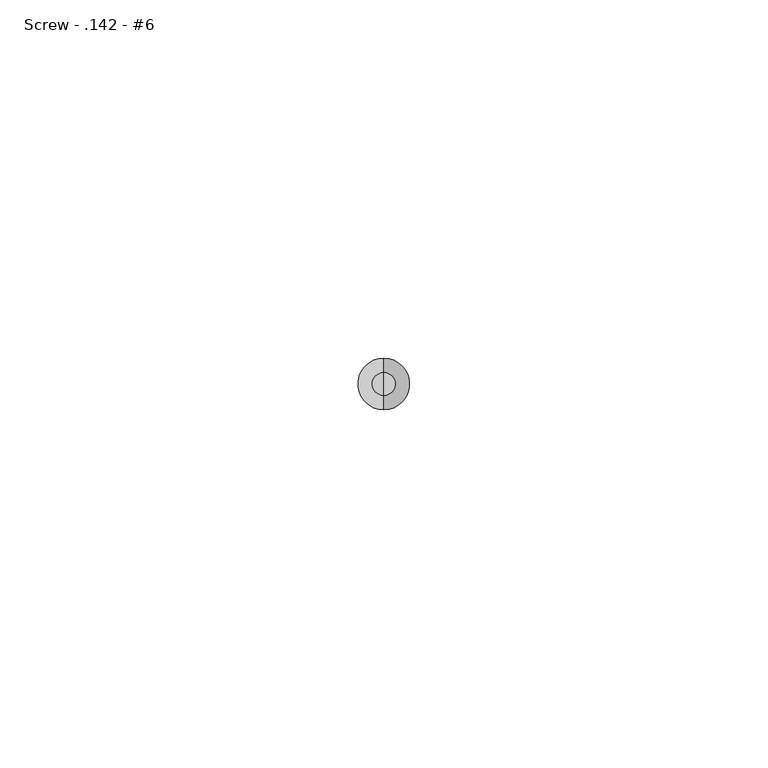
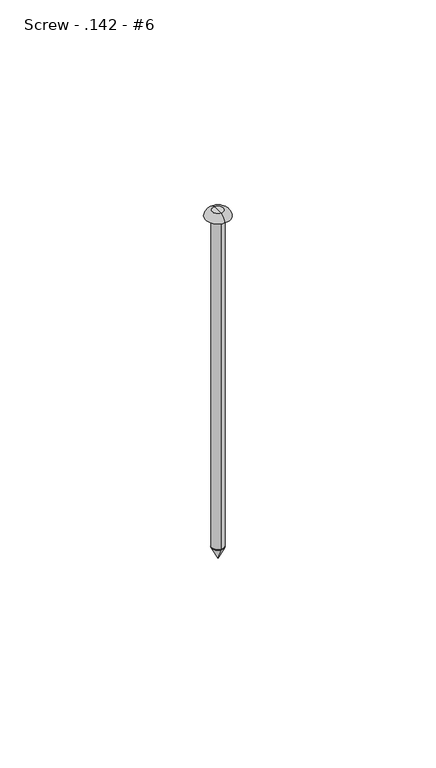
"""IFC4 building model written with IfcOpenShell, lengths in millimetres: fastener geometry, 060523 - W_P_C - Fastenings - Generic : Screw - .142 - #6."""

from ifc_helpers import new_model, si_unit, point, frame, origin, origin_2d, place, context, project, spatial, polyline, circle_curve, ellipse_curve, trimmed, segment, composite_curve, outline, extrude, source, transform, mapped, element, save
from ifc_brep_helpers import plane_surface, revolved_surface, advanced_brep


def screw_142_6_6657c1da(model_context):
    return source(origin(), model_context, "Body", "SolidModel", [
        advanced_brep(
        [(0.0, -1.8034, -101.6), (0.0, 1.8034, -101.6), (0.0, 0.0, -101.6), (0.0, 0.0, -105.2068)],
        [
            (0, 1, circle_curve(frame((0.0, 0.0, -101.6), z_axis=(0.0, 0.0, 1.0), x_axis=(0.0, 1.0, 0.0)), 1.8034)),
            (1, 2),
            (2, 0),
            (1, 0, circle_curve(frame((0.0, 0.0, -101.6), z_axis=(0.0, 0.0, 1.0), x_axis=(0.0, 1.0, 0.0)), 1.8034)),
            (3, 1),
            (0, 3),
        ],
        [
            plane_surface(frame((0.0, 0.0, -101.6), z_axis=(0.0, 0.0, 1.0), x_axis=(0.0, 1.0, 0.0))),
            revolved_surface(polyline([(0.0, 1.8034, -101.6), (0.0, 0.0, -105.2068)]), (0.0, 0.0, -103.0840259), (0.0, 0.0, -1.0)),
        ],
        [
            (0, [[1, 2, 3]]),
            (0, [[4, -3, -2]]),
            (1, [[5, -1, 6]]),
            (1, [[-6, -4, -5]]),
        ],
    ),
        advanced_brep(
        [(0.0, 3.6068, 0.0), (0.0, -3.6068, 0.0), (0.0, 0.0, 0.0), (0.0, 0.0, 1.8034), (0.0, -1.5875, 1.8034), (0.0, 1.5875, 1.8034)],
        [
            (0, 1, circle_curve(frame((0.0, 0.0, 0.0), z_axis=(0.0, 0.0, -1.0), x_axis=(0.0, -1.0, 0.0)), 3.6068)),
            (1, 2),
            (2, 0),
            (1, 0, circle_curve(frame((0.0, 0.0, 0.0), z_axis=(0.0, 0.0, -1.0), x_axis=(0.0, -1.0, 0.0)), 3.6068)),
            (3, 4),
            (4, 5, circle_curve(frame((0.0, 0.0, 1.8034), z_axis=(0.0, 0.0, 1.0), x_axis=(0.0, -1.0, 0.0)), 1.5875)),
            (5, 3),
            (5, 4, circle_curve(frame((0.0, 0.0, 1.8034), z_axis=(0.0, 0.0, 1.0), x_axis=(0.0, -1.0, 0.0)), 1.5875)),
            (4, 1, circle_curve(frame((0.0, -1.5875, -0.2288236), z_axis=(1.0, 0.0, 0.0), x_axis=(0.0, -1.0, 0.0)), 2.0322236)),
            (0, 5, circle_curve(frame((0.0, 1.5875, -0.2288236), z_axis=(1.0, 0.0, 0.0), x_axis=(0.0, 1.0, 0.0)), 2.0322236)),
        ],
        [
            plane_surface(frame((0.0, 0.0, 0.0), z_axis=(0.0, 0.0, -1.0), x_axis=(0.0, -1.0, 0.0))),
            plane_surface(frame((0.0, 0.0, 1.8034), z_axis=(0.0, 0.0, 1.0), x_axis=(0.0, -1.0, 0.0))),
            revolved_surface(trimmed(ellipse_curve(frame((0.0, -1.5875, -0.2288236), z_axis=(-1.0, 0.0, 0.0), x_axis=(0.0, -1.0, 0.0)), 2.0322236, 2.0322236), [point((0.0, -3.6068, 0.0))], [point((0.0, -1.5875, 1.8034))], True, "CARTESIAN"), (0.0, 0.0, 1.4840259), (0.0, 0.0, 1.0)),
        ],
        [
            (0, [[1, 2, 3]]),
            (0, [[4, -3, -2]]),
            (1, [[5, 6, 7]]),
            (1, [[-7, 8, -5]]),
            (2, [[-6, 9, -1, 10]]),
            (2, [[-8, -10, -4, -9]]),
        ],
    ),
        extrude(outline(composite_curve([segment(trimmed(circle_curve(origin_2d(), 1.8034), [point((0.0, -1.8034))], [point((0.0, 1.8034))], False, "CARTESIAN"), True, "CONTINUOUS"), segment(trimmed(circle_curve(origin_2d(), 1.8034), [point((0.0, 1.8034))], [point((0.0, -1.8034))], False, "CARTESIAN"), True, "CONTINUOUS")], self_intersect=False)), frame((0.0, 0.0, -101.6), z_axis=(0.0, 0.0, 1.0), x_axis=(1.0, 0.0, 0.0)), (0.0, 0.0, 1.0), 101.6),
    ])


if __name__ == "__main__":
    model = new_model("IFC4")
    model_context = context("Model", 3, world=origin())
    ifc_project = project(units=[si_unit("LENGTHUNIT", "METRE", prefix="MILLI")], contexts=[model_context])
    site = spatial("IfcSite", under=ifc_project)
    building = spatial("IfcBuilding", under=site)
    placement = place(None, origin())
    screw_142_6_shape = screw_142_6_6657c1da(model_context)
    element("IfcFastener", 1, ObjectType="060523 - W_P_C - Fastenings - Generic : Screw - .142 - #6", at=placement, inside=building, context=model_context, shape_type="MappedRepresentation", body=[
        mapped(screw_142_6_shape, transform((0.0, 0.0, 0.0), x_axis=(1.0, 0.0, 0.0), y_axis=(0.0, 1.0, 0.0), z_axis=(0.0, 0.0, 1.0))),
    ])
    save(model, "model.ifc")

# Revit data of these elements
# Type "060523 - W_P_C - Fastenings - Generic : Screw - .142 - #6"
#   Washer_Thickness = 0' - 0.00333"
#   Washer Radius = 0' - 0.081"
#   Washer Offset - Head = 0' - 0"
#   Washer Offset = 0' - 0"
#   Thickness_of_Substrate [instance default] = 0' - 1"
#   Side = 0' - 0 37/64"
#   Radius = 0' - 0.071"
#   Length [instance default] = 0' - 4"
#   Head Size = 0' - 1"
#   Head Radius = 0' - 0 1/2"
#   Head Height = 0' - 0.01"
#   Double Diameter = 0' - 0.284"
#   Diameter = 0' - 0.142"
#   Default Elevation = 4' - 0"
#   Washer_Nut_Visibility = no
#   Washer_Head_Visibility = no
#   Round_Head_Visibility = yes
#   Point Visibility = yes
#   Nut_Visibility = no
#   Hex_Head_Visiblilty = no
#   Washer Material = none
#   Bolt Material (Size) = AT SILL - FASTENER AT 24" O.C.
# Element 1 (IfcFastener, "060523 - W_P_C - Fastenings - Generic : Screw - .142 - #6")
#   Materials on its faces: "AT SILL - FASTENER AT 24\" O.C."
# Materials
#   "AT SILL - FASTENER AT 24\" O.C.": class "Generic", colour RGB 120 120 120, transparency 0, Cost = 0
